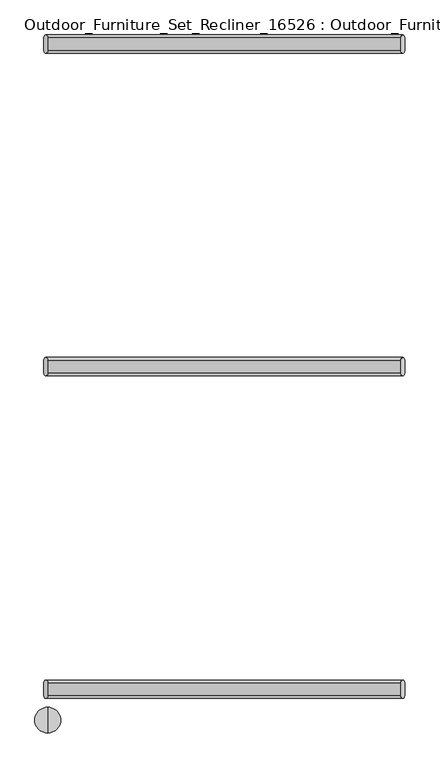
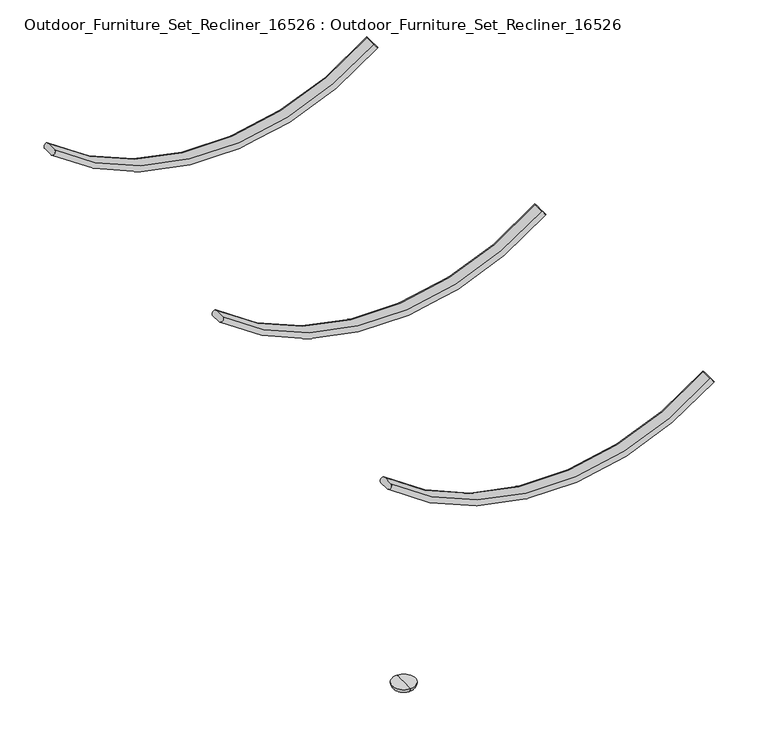
"""IFC4 building model written with IfcOpenShell, lengths in millimetres: furniture geometry, Outdoor_Furniture_Set_Recliner_16526 : Outdoor_Furniture_Set_Recliner_16526."""

from ifc_helpers import new_model, si_unit, point, frame, origin, place, context, project, spatial, polyline, circle_curve, ellipse_curve, trimmed, source, transform, mapped, element, save
from ifc_brep_helpers import plane_surface, cylinder_surface, revolved_surface, advanced_brep


def outdoor_furniture_set_recliner_16526_outdoor_furniture_set_6b74ba21(model_context):
    return source(origin(), model_context, "Body", "AdvancedBrep", [
        advanced_brep(
        [(287.5, -215.0, 363.125), (287.5, -235.0, 363.125), (293.9447261, -235.0, 355.4787261), (293.9447261, -215.0, 355.4787261), (-287.5, -215.0, 363.125), (-293.9447261, -215.0, 355.4787261), (-293.9447261, -235.0, 355.4787261), (-287.5, -235.0, 363.125)],
        [
            (0, 1),
            (1, 2, circle_curve(frame((290.7223631, -235.0, 359.301863), z_axis=(0.7646273934226512, 0.0, 0.6444726132487572), x_axis=(0.6444726132487572, 0.0, -0.7646273934226512)), 5.0)),
            (2, 3),
            (3, 0, circle_curve(frame((290.7223631, -215.0, 359.301863), z_axis=(0.7646273934226512, 0.0, 0.6444726132487572), x_axis=(0.6444726132487572, 0.0, -0.7646273934226512)), 5.0)),
            (4, 5, circle_curve(frame((-290.7223631, -215.0, 359.301863), z_axis=(-0.7646273934226475, 0.0, 0.6444726132487614), x_axis=(-0.6444726132487614, 0.0, -0.7646273934226475)), 5.0)),
            (5, 6),
            (6, 7, circle_curve(frame((-290.7223631, -235.0, 359.301863), z_axis=(-0.7646273934226475, 0.0, 0.6444726132487614), x_axis=(-0.6444726132487614, 0.0, -0.7646273934226475)), 5.0)),
            (7, 4),
            (7, 1, circle_curve(frame((0.0, -235.0, 704.2261905), z_axis=(0.0, -1.0, 0.0), x_axis=(0.6444726132487572, 0.0, -0.7646273934226512)), 446.1011905)),
            (0, 4, circle_curve(frame((0.0, -215.0, 704.2261905), z_axis=(0.0, 1.0, 0.0), x_axis=(0.6444726132487572, 0.0, -0.7646273934226512)), 446.1011905)),
            (6, 2, circle_curve(frame((0.0, -235.0, 704.2261905), z_axis=(0.0, -1.0, 0.0), x_axis=(0.6444726132487572, 0.0, -0.7646273934226512)), 456.1011905)),
            (5, 3, circle_curve(frame((0.0, -215.0, 704.2261905), z_axis=(0.0, -1.0, 0.0), x_axis=(0.6444726132487572, 0.0, -0.7646273934226512)), 456.1011905)),
        ],
        [
            plane_surface(frame((287.5, -225.0, 363.125), z_axis=(0.7646273934226512, 0.0, 0.6444726132487572), x_axis=(0.0, -1.0, 0.0))),
            plane_surface(frame((-287.5, -225.0, 363.125), z_axis=(-0.7646273934226476, 0.0, 0.6444726132487615), x_axis=(0.0, -1.0, 0.0))),
            revolved_surface(polyline([(287.5000000149166, -215.0, 363.12500000524346), (287.5000000149166, -235.0, 363.12500000524346)]), (0.0, -225.0, 704.2261905), (0.0, 1.0, 0.0)),
            revolved_surface(trimmed(ellipse_curve(frame((290.7223631, -235.0, 359.301863), z_axis=(0.7646273934226512, 0.0, 0.6444726132487572), x_axis=(0.6444726132487572, 0.0, -0.7646273934226512)), 5.0, 5.0), [point((287.5, -235.0, 363.125))], [point((293.9447261, -235.0, 355.4787261))], True, "CARTESIAN"), (0.0, -225.0, 704.2261905), (0.0, 1.0, 0.0)),
            cylinder_surface(frame((0.0, -225.0, 704.2261905), z_axis=(0.0, 1.0, 0.0), x_axis=(0.6444726132487572, 0.0, -0.7646273934226512)), 456.1011905),
            revolved_surface(trimmed(ellipse_curve(frame((290.7223631, -215.0, 359.301863), z_axis=(0.7646273934226512, 0.0, 0.6444726132487572), x_axis=(0.6444726132487572, 0.0, -0.7646273934226512)), 5.0, 5.0), [point((293.9447261, -215.0, 355.4787261))], [point((287.5, -215.0, 363.125))], True, "CARTESIAN"), (0.0, -225.0, 704.2261905), (0.0, 1.0, 0.0)),
        ],
        [
            (0, [[1, 2, 3, 4]]),
            (1, [[5, 6, 7, 8]]),
            (2, [[9, -1, 10, -8]]),
            (3, [[11, -2, -9, -7]]),
            (4, [[12, -3, -11, -6]]),
            (5, [[-10, -4, -12, -5]]),
        ],
    ),
        advanced_brep(
        [(287.5, 310.0, 363.125), (287.5, 290.0, 363.125), (293.9447261, 290.0, 355.4787261), (293.9447261, 310.0, 355.4787261), (-287.5, 310.0, 363.125), (-293.9447261, 310.0, 355.4787261), (-293.9447261, 290.0, 355.4787261), (-287.5, 290.0, 363.125)],
        [
            (0, 1),
            (1, 2, circle_curve(frame((290.7223631, 290.0, 359.301863), z_axis=(0.7646273934226512, 0.0, 0.6444726132487572), x_axis=(0.6444726132487572, 0.0, -0.7646273934226512)), 5.0)),
            (2, 3),
            (3, 0, circle_curve(frame((290.7223631, 310.0, 359.301863), z_axis=(0.7646273934226512, 0.0, 0.6444726132487572), x_axis=(0.6444726132487572, 0.0, -0.7646273934226512)), 5.0)),
            (4, 5, circle_curve(frame((-290.7223631, 310.0, 359.301863), z_axis=(-0.7646273934226475, 0.0, 0.6444726132487614), x_axis=(-0.6444726132487614, 0.0, -0.7646273934226475)), 5.0)),
            (5, 6),
            (6, 7, circle_curve(frame((-290.7223631, 290.0, 359.301863), z_axis=(-0.7646273934226475, 0.0, 0.6444726132487614), x_axis=(-0.6444726132487614, 0.0, -0.7646273934226475)), 5.0)),
            (7, 4),
            (7, 1, circle_curve(frame((0.0, 290.0, 704.2261905), z_axis=(0.0, -1.0, 0.0), x_axis=(0.6444726132487572, 0.0, -0.7646273934226512)), 446.1011905)),
            (0, 4, circle_curve(frame((0.0, 310.0, 704.2261905), z_axis=(0.0, 1.0, 0.0), x_axis=(0.6444726132487572, 0.0, -0.7646273934226512)), 446.1011905)),
            (6, 2, circle_curve(frame((0.0, 290.0, 704.2261905), z_axis=(0.0, -1.0, 0.0), x_axis=(0.6444726132487572, 0.0, -0.7646273934226512)), 456.1011905)),
            (5, 3, circle_curve(frame((0.0, 310.0, 704.2261905), z_axis=(0.0, -1.0, 0.0), x_axis=(0.6444726132487572, 0.0, -0.7646273934226512)), 456.1011905)),
        ],
        [
            plane_surface(frame((287.5, 300.0, 363.125), z_axis=(0.7646273934226512, 0.0, 0.6444726132487572), x_axis=(0.0, -1.0, 0.0))),
            plane_surface(frame((-287.5, 300.0, 363.125), z_axis=(-0.7646273934226476, 0.0, 0.6444726132487615), x_axis=(0.0, -1.0, 0.0))),
            revolved_surface(polyline([(287.5000000149166, 310.0, 363.12500000524346), (287.5000000149166, 290.0, 363.12500000524346)]), (0.0, 300.0, 704.2261905), (0.0, 1.0, 0.0)),
            revolved_surface(trimmed(ellipse_curve(frame((290.7223631, 290.0, 359.301863), z_axis=(0.7646273934226512, 0.0, 0.6444726132487572), x_axis=(0.6444726132487572, 0.0, -0.7646273934226512)), 5.0, 5.0), [point((287.5, 290.0, 363.125))], [point((293.9447261, 290.0, 355.4787261))], True, "CARTESIAN"), (0.0, 300.0, 704.2261905), (0.0, 1.0, 0.0)),
            cylinder_surface(frame((0.0, 300.0, 704.2261905), z_axis=(0.0, 1.0, 0.0), x_axis=(0.6444726132487572, 0.0, -0.7646273934226512)), 456.1011905),
            revolved_surface(trimmed(ellipse_curve(frame((290.7223631, 310.0, 359.301863), z_axis=(0.7646273934226512, 0.0, 0.6444726132487572), x_axis=(0.6444726132487572, 0.0, -0.7646273934226512)), 5.0, 5.0), [point((293.9447261, 310.0, 355.4787261))], [point((287.5, 310.0, 363.125))], True, "CARTESIAN"), (0.0, 300.0, 704.2261905), (0.0, 1.0, 0.0)),
        ],
        [
            (0, [[1, 2, 3, 4]]),
            (1, [[5, 6, 7, 8]]),
            (2, [[9, -1, 10, -8]]),
            (3, [[11, -2, -9, -7]]),
            (4, [[12, -3, -11, -6]]),
            (5, [[-10, -4, -12, -5]]),
        ],
    ),
        advanced_brep(
        [(287.5, -740.0, 363.125), (287.5, -760.0, 363.125), (293.9447261, -760.0, 355.4787261), (293.9447261, -740.0, 355.4787261), (-287.5, -740.0, 363.125), (-293.9447261, -740.0, 355.4787261), (-293.9447261, -760.0, 355.4787261), (-287.5, -760.0, 363.125)],
        [
            (0, 1),
            (1, 2, circle_curve(frame((290.7223631, -760.0, 359.301863), z_axis=(0.7646273934226512, 0.0, 0.6444726132487572), x_axis=(0.6444726132487572, 0.0, -0.7646273934226512)), 5.0)),
            (2, 3),
            (3, 0, circle_curve(frame((290.7223631, -740.0, 359.301863), z_axis=(0.7646273934226512, 0.0, 0.6444726132487572), x_axis=(0.6444726132487572, 0.0, -0.7646273934226512)), 5.0)),
            (4, 5, circle_curve(frame((-290.7223631, -740.0, 359.301863), z_axis=(-0.7646273934226475, 0.0, 0.6444726132487614), x_axis=(-0.6444726132487614, 0.0, -0.7646273934226475)), 5.0)),
            (5, 6),
            (6, 7, circle_curve(frame((-290.7223631, -760.0, 359.301863), z_axis=(-0.7646273934226475, 0.0, 0.6444726132487614), x_axis=(-0.6444726132487614, 0.0, -0.7646273934226475)), 5.0)),
            (7, 4),
            (7, 1, circle_curve(frame((0.0, -760.0, 704.2261905), z_axis=(0.0, -1.0, 0.0), x_axis=(0.6444726132487572, 0.0, -0.7646273934226512)), 446.1011905)),
            (0, 4, circle_curve(frame((0.0, -740.0, 704.2261905), z_axis=(0.0, 1.0, 0.0), x_axis=(0.6444726132487572, 0.0, -0.7646273934226512)), 446.1011905)),
            (6, 2, circle_curve(frame((0.0, -760.0, 704.2261905), z_axis=(0.0, -1.0, 0.0), x_axis=(0.6444726132487572, 0.0, -0.7646273934226512)), 456.1011905)),
            (5, 3, circle_curve(frame((0.0, -740.0, 704.2261905), z_axis=(0.0, -1.0, 0.0), x_axis=(0.6444726132487572, 0.0, -0.7646273934226512)), 456.1011905)),
        ],
        [
            plane_surface(frame((287.5, -750.0, 363.125), z_axis=(0.7646273934226512, 0.0, 0.6444726132487572), x_axis=(0.0, -1.0, 0.0))),
            plane_surface(frame((-287.5, -750.0, 363.125), z_axis=(-0.7646273934226476, 0.0, 0.6444726132487615), x_axis=(0.0, -1.0, 0.0))),
            revolved_surface(polyline([(287.5000000149166, -740.0, 363.12500000524346), (287.5000000149166, -760.0, 363.12500000524346)]), (0.0, -750.0, 704.2261905), (0.0, 1.0, 0.0)),
            revolved_surface(trimmed(ellipse_curve(frame((290.7223631, -760.0, 359.301863), z_axis=(0.7646273934226512, 0.0, 0.6444726132487572), x_axis=(0.6444726132487572, 0.0, -0.7646273934226512)), 5.0, 5.0), [point((287.5, -760.0, 363.125))], [point((293.9447261, -760.0, 355.4787261))], True, "CARTESIAN"), (0.0, -750.0, 704.2261905), (0.0, 1.0, 0.0)),
            cylinder_surface(frame((0.0, -750.0, 704.2261905), z_axis=(0.0, 1.0, 0.0), x_axis=(0.6444726132487572, 0.0, -0.7646273934226512)), 456.1011905),
            revolved_surface(trimmed(ellipse_curve(frame((290.7223631, -740.0, 359.301863), z_axis=(0.7646273934226512, 0.0, 0.6444726132487572), x_axis=(0.6444726132487572, 0.0, -0.7646273934226512)), 5.0, 5.0), [point((293.9447261, -740.0, 355.4787261))], [point((287.5, -740.0, 363.125))], True, "CARTESIAN"), (0.0, -750.0, 704.2261905), (0.0, 1.0, 0.0)),
        ],
        [
            (0, [[1, 2, 3, 4]]),
            (1, [[5, 6, 7, 8]]),
            (2, [[9, -1, 10, -8]]),
            (3, [[11, -2, -9, -7]]),
            (4, [[12, -3, -11, -6]]),
            (5, [[-10, -4, -12, -5]]),
        ],
    ),
        advanced_brep(
        [(-287.75, -821.375, 10.0), (-287.75, -800.375, 10.0), (-287.75, -790.0, 10.0), (-287.75, -784.2697293, 10.0), (-287.75, -779.375, 10.0), (-301.2266559, -784.2697293, 10.0), (-306.0081317, -790.0, 10.0), (-269.4918683, -790.0, 10.0), (-274.2733441, -784.2697293, 10.0), (-287.75, -811.375, 0.0), (-287.75, -789.375, 0.0), (-287.75, -800.375, 0.0)],
        [
            (0, 1),
            (1, 2),
            (2, 3),
            (3, 4),
            (4, 5, circle_curve(frame((-287.75, -800.375, 10.0), z_axis=(0.0, 0.0, 1.0), x_axis=(0.0, 1.0, 0.0)), 21.0)),
            (5, 6, circle_curve(frame((-287.75, -800.375, 10.0), z_axis=(0.0, 0.0, 1.0), x_axis=(0.0, 1.0, 0.0)), 21.0)),
            (6, 0, circle_curve(frame((-287.75, -800.375, 10.0), z_axis=(0.0, 0.0, 1.0), x_axis=(0.0, 1.0, 0.0)), 21.0)),
            (0, 7, circle_curve(frame((-287.75, -800.375, 10.0), z_axis=(0.0, 0.0, 1.0), x_axis=(0.0, 1.0, 0.0)), 21.0)),
            (7, 8, circle_curve(frame((-287.75, -800.375, 10.0), z_axis=(0.0, 0.0, 1.0), x_axis=(0.0, 1.0, 0.0)), 21.0)),
            (8, 4, circle_curve(frame((-287.75, -800.375, 10.0), z_axis=(0.0, 0.0, 1.0), x_axis=(0.0, 1.0, 0.0)), 21.0)),
            (9, 10, circle_curve(frame((-287.75, -800.375, 0.0), z_axis=(0.0, 0.0, -1.0), x_axis=(0.0, 1.0, 0.0)), 11.0)),
            (10, 11),
            (11, 9),
            (10, 9, circle_curve(frame((-287.75, -800.375, 0.0), z_axis=(0.0, 0.0, -1.0), x_axis=(0.0, 1.0, 0.0)), 11.0)),
            (9, 0, circle_curve(frame((-287.75, -811.375, 10.0), z_axis=(-1.0, 0.0, 0.0), x_axis=(0.0, -1.0, 0.0)), 10.0)),
            (4, 10, circle_curve(frame((-287.75, -789.375, 10.0), z_axis=(-1.0, 0.0, 0.0), x_axis=(0.0, 1.0, 0.0)), 10.0)),
        ],
        [
            plane_surface(frame((-287.75, -800.375, 10.0), z_axis=(0.0, 0.0, 1.0), x_axis=(0.0, 1.0, 0.0))),
            plane_surface(frame((-287.75, -800.375, 0.0), z_axis=(0.0, 0.0, -1.0), x_axis=(0.0, 1.0, 0.0))),
            revolved_surface(trimmed(ellipse_curve(frame((-287.75, -789.375, 10.0), z_axis=(1.0, 0.0, 0.0), x_axis=(0.0, 1.0, 0.0)), 10.0, 10.0), [point((-287.75, -789.375, 0.0))], [point((-287.75, -779.375, 10.0))], True, "CARTESIAN"), (-287.75, -800.375, 0.0), (0.0, 0.0, 1.0)),
        ],
        [
            (0, [[1, 2, 3, 4, 5, 6, 7]]),
            (0, [[-1, 8, 9, 10, -4, -3, -2]]),
            (1, [[11, 12, 13]]),
            (1, [[-12, 14, -13]]),
            (2, [[-11, 15, -7, -6, -5, 16]]),
            (2, [[-14, -16, -10, -9, -8, -15]]),
        ],
    ),
    ])


if __name__ == "__main__":
    model = new_model("IFC4")
    model_context = context("Model", 3, world=origin())
    ifc_project = project(units=[si_unit("LENGTHUNIT", "METRE", prefix="MILLI")], contexts=[model_context])
    site = spatial("IfcSite", under=ifc_project)
    building = spatial("IfcBuilding", under=site)
    placement = place(None, origin())
    outdoor_furniture_set_recliner_16526_outdoor_furniture_set_shape = outdoor_furniture_set_recliner_16526_outdoor_furniture_set_6b74ba21(model_context)
    element("IfcFurniture", 1, ObjectType="Outdoor_Furniture_Set_Recliner_16526 : Outdoor_Furniture_Set_Recliner_16526", at=placement, inside=building, context=model_context, shape_type="MappedRepresentation", body=[
        mapped(outdoor_furniture_set_recliner_16526_outdoor_furniture_set_shape, transform((0.0, 0.0, 0.0), x_axis=(1.0, 0.0, 0.0), y_axis=(0.0, 1.0, 0.0), z_axis=(0.0, 0.0, 1.0))),
    ])
    save(model, "model.ifc")

# Revit data of these elements
# Type "Outdoor_Furniture_Set_Recliner_16526 : Outdoor_Furniture_Set_Recliner_16526"
#   Back Angle [instance default] = 25.00°
#   Frame Material = Furniture - Paint - White Gloss
#   Fabric Material = Furniture - Fabric - White Canvas
#   Assembly Code = ""
# Element 1 (IfcFurniture, "Outdoor_Furniture_Set_Recliner_16526 : Outdoor_Furniture_Set_Recliner_16526")
#   Materials on its faces: "Furniture - Paint - White Gloss", "Furniture - Fabric - White Canvas", "Furniture - Rubber - Black"
# Materials
#   "Furniture - Paint - White Gloss": class "Paint", colour RGB 255 255 255, transparency 0
#   "Furniture - Fabric - White Canvas": class "Fabric", colour RGB 255 255 255, transparency 0.1
#   "Furniture - Rubber - Black": class "Paint", colour RGB 127 127 127, transparency 0
